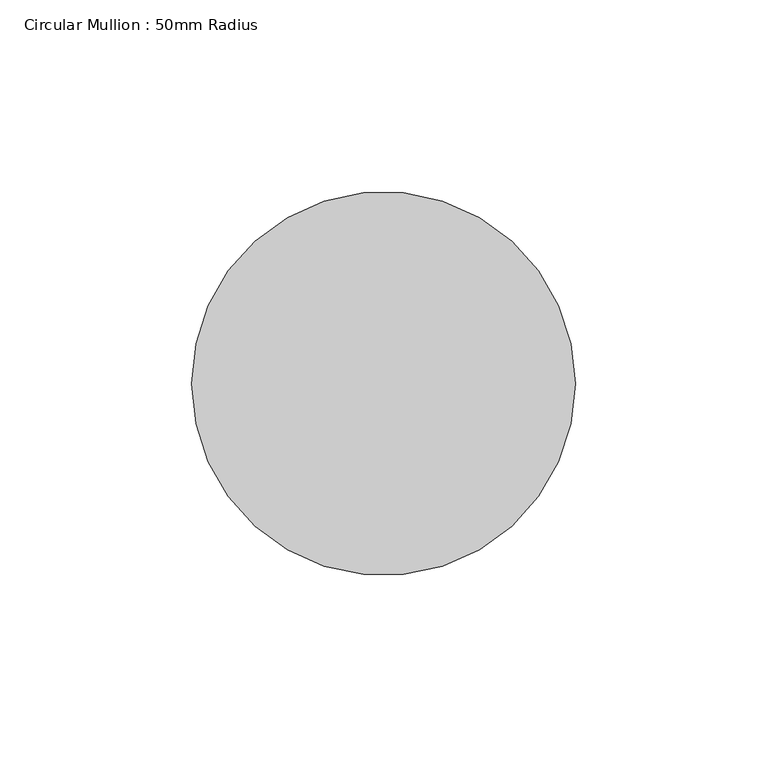
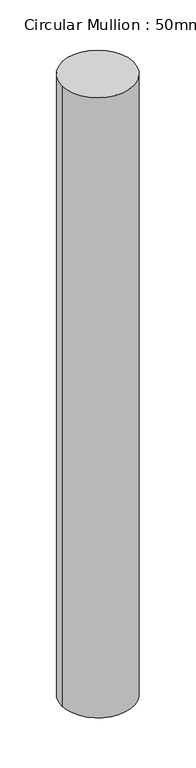
"""IFC4 building model written with IfcOpenShell, lengths in millimetres: member geometry, Circular Mullion : 50mm Radius."""

import ifcopenshell
import ifcopenshell.guid

model = None  # the IFC model being written
_history = None  # IfcOwnerHistory: only IFC2X3 demands one
_inside = {}  # id of a spatial element -> (the spatial element, [elements in it])
_under = {}  # id of a project, library or spatial element -> (it, [spatial elements below it])
_declared = {}  # id of a project -> (the project, [libraries it declares])
_typed = {}  # id of a type object -> (the type object, [elements of that type])
_made_of = {}  # id of a material, layer set ... -> (it, [elements and type objects made of it])


def new_model(schema):
    """Start an empty IFC model of exactly this schema.

    Asked for "IFC4X3", IfcOpenShell would pick the latest addendum, in which some entities
    have other attributes; the version numbers below select the first issue.
    IFC2X3 requires an IfcOwnerHistory on every rooted entity: one is made here for all.
    """
    global model, _history
    if schema == "IFC4X3":
        model = ifcopenshell.file(schema_version=(4, 3, 0, 0))
    else:
        model = ifcopenshell.file(schema=schema)
    _inside.clear()
    _under.clear()
    _declared.clear()
    _typed.clear()
    _made_of.clear()
    _history = None
    if model.schema == "IFC2X3":
        org = make("IfcOrganization", Name="unknown")
        user = make(
            "IfcPersonAndOrganization",
            ThePerson=make("IfcPerson", FamilyName="unknown"),
            TheOrganization=org,
        )
        app = make(
            "IfcApplication",
            ApplicationDeveloper=org,
            Version="unknown",
            ApplicationFullName="unknown",
            ApplicationIdentifier="unknown",
        )
        _history = make(
            "IfcOwnerHistory",
            OwningUser=user,
            OwningApplication=app,
            ChangeAction="ADDED",
            CreationDate=0,
        )
    return model


def make(cls, **values):
    """One entity of the class cls with the attributes given. An attribute that is None is left unset."""
    return model.create_entity(
        cls, **{name: value for name, value in values.items() if value is not None}
    )


def rooted(cls, **values):
    """An entity with a GlobalId (a new one), such as an element, a storey or a relation."""
    return make(cls, GlobalId=ifcopenshell.guid.new(), OwnerHistory=_history, **values)


def si_unit(unit_type, name, prefix=None):
    """IfcSIUnit, for example si_unit("LENGTHUNIT", "METRE", prefix="MILLI")."""
    return make("IfcSIUnit", UnitType=unit_type, Prefix=prefix, Name=name)


def assignment(units):
    """IfcUnitAssignment: the units of a project."""
    return None if units is None else make("IfcUnitAssignment", Units=units)


def point(xyz):
    """IfcCartesianPoint."""
    return None if xyz is None else make("IfcCartesianPoint", Coordinates=xyz)


def direction(xyz):
    """IfcDirection."""
    return None if xyz is None else make("IfcDirection", DirectionRatios=xyz)


def frame(location, z_axis=None, x_axis=None):
    """IfcAxis2Placement3D, a coordinate frame: its origin and axes. An axis left out is left unset."""
    return make(
        "IfcAxis2Placement3D",
        Location=point(location),
        Axis=direction(z_axis),
        RefDirection=direction(x_axis),
    )


def frame_2d(location, x_axis=None):
    """IfcAxis2Placement2D, a coordinate frame in the plane: its origin and x axis."""
    return make(
        "IfcAxis2Placement2D", Location=point(location), RefDirection=direction(x_axis)
    )


def origin():
    """The frame at (0, 0, 0) with its axes left unset."""
    return frame((0.0, 0.0, 0.0))


def origin_2d():
    """The frame at (0, 0) in the plane with its x axis left unset."""
    return frame_2d((0.0, 0.0))


def place(relative_to, where):
    """IfcLocalPlacement: puts the frame where relative to a parent placement (None: the world)."""
    return make(
        "IfcLocalPlacement", PlacementRelTo=relative_to, RelativePlacement=where
    )


def context(
    kind, dimensions, precision=None, world=None, true_north=None, identifier=None
):
    """IfcGeometricRepresentationContext, for example the 3D "Model" context."""
    return make(
        "IfcGeometricRepresentationContext",
        ContextIdentifier=identifier,
        ContextType=kind,
        CoordinateSpaceDimension=dimensions,
        Precision=precision,
        WorldCoordinateSystem=world,
        TrueNorth=true_north,
    )


def project(units=None, contexts=None):
    """IfcProject with its units and contexts."""
    return rooted(
        "IfcProject",
        Name="project",
        RepresentationContexts=contexts,
        UnitsInContext=assignment(units),
    )


def spatial(cls, under=None, at=None, **own):
    """A site, building, storey or space (cls), placed at a placement, below another one or the project."""
    s = rooted(cls, ObjectPlacement=at, **own)
    if under is not None:
        _under.setdefault(under.id(), (under, []))[1].append(s)
    return s


def circle_curve(where, radius):
    """IfcCircle in the frame where."""
    return make("IfcCircle", Position=where, Radius=radius)


def trimmed(basis, trim1, trim2, sense, master):
    """IfcTrimmedCurve: the piece of a basis curve between two trims."""
    return make(
        "IfcTrimmedCurve",
        BasisCurve=basis,
        Trim1=trim1,
        Trim2=trim2,
        SenseAgreement=sense,
        MasterRepresentation=master,
    )


def segment(curve, same_sense, transition):
    """IfcCompositeCurveSegment."""
    return make(
        "IfcCompositeCurveSegment",
        Transition=transition,
        SameSense=same_sense,
        ParentCurve=curve,
    )


def composite_curve(segments, self_intersect=None):
    """IfcCompositeCurve: segments joined end to end."""
    return make("IfcCompositeCurve", Segments=segments, SelfIntersect=self_intersect)


def outline(outer, holes=None, kind="AREA"):
    """IfcArbitraryClosedProfileDef: a profile drawn as a closed curve; with holes, ...WithVoids."""
    if holes is None:
        return make("IfcArbitraryClosedProfileDef", ProfileType=kind, OuterCurve=outer)
    return make(
        "IfcArbitraryProfileDefWithVoids",
        ProfileType=kind,
        OuterCurve=outer,
        InnerCurves=holes,
    )


def extrude(swept, where, along, depth):
    """IfcExtrudedAreaSolid: the profile swept, set in the frame where, extruded along a direction by depth."""
    return make(
        "IfcExtrudedAreaSolid",
        SweptArea=swept,
        Position=where,
        ExtrudedDirection=direction(along),
        Depth=depth,
    )


def shape(context_of_items, identifier, shape_type, items):
    """IfcShapeRepresentation: the items that make up one representation, for example the "Body"."""
    return make(
        "IfcShapeRepresentation",
        ContextOfItems=context_of_items,
        RepresentationIdentifier=identifier,
        RepresentationType=shape_type,
        Items=items,
    )


def source(mapping_origin, context_of_items, identifier, shape_type, items):
    """IfcRepresentationMap: a shape defined once, which mapped items show again and again."""
    return make(
        "IfcRepresentationMap",
        MappingOrigin=mapping_origin,
        MappedRepresentation=shape(context_of_items, identifier, shape_type, items),
    )


def transform(
    local_origin,
    x_axis=None,
    y_axis=None,
    z_axis=None,
    scale=None,
    scale2=None,
    scale3=None,
    uniform=True,
):
    """IfcCartesianTransformationOperator3D, or its non-uniform kind. x_axis, y_axis, z_axis: its Axis1, 2, 3."""
    if uniform:
        return make(
            "IfcCartesianTransformationOperator3D",
            Axis1=direction(x_axis),
            Axis2=direction(y_axis),
            LocalOrigin=point(local_origin),
            Scale=scale,
            Axis3=direction(z_axis),
        )
    return make(
        "IfcCartesianTransformationOperator3DnonUniform",
        Axis1=direction(x_axis),
        Axis2=direction(y_axis),
        LocalOrigin=point(local_origin),
        Scale=scale,
        Axis3=direction(z_axis),
        Scale2=scale2,
        Scale3=scale3,
    )


def mapped(mapping_source, mapping_target):
    """IfcMappedItem: shows the shape of a source again, moved by a transform."""
    return make(
        "IfcMappedItem", MappingSource=mapping_source, MappingTarget=mapping_target
    )


def made_of(thing, what):
    """Note that an element or type object is made of a material, layer set ...; save() writes the relation."""
    if what is not None:
        _made_of.setdefault(what.id(), (what, []))[1].append(thing)
    return thing


def element(
    cls,
    number,
    at=None,
    inside=None,
    cuts=None,
    type_object=None,
    material=None,
    context=None,
    identifier="Body",
    shape_type=None,
    held_by="IfcProductDefinitionShape",
    body=None,
    shapes=None,
    **own,
):
    """One element of the class cls, such as IfcWall. Its Tag is "e" and its number.

    at: its placement. inside: the storey or other place that contains it. cuts: it is an
    opening in that element (IfcRelVoidsElement). A single representation is given by context,
    identifier, shape_type and body (its items); several are given by shapes. held_by: the class
    of the entity that holds the representations. save() writes the other relations.
    """
    e = rooted(cls, Tag="e%d" % number, ObjectPlacement=at, **own)
    if body is not None:
        shapes = [shape(context, identifier, shape_type, body)]
    if shapes is not None:
        e.Representation = make(held_by, Representations=shapes)
    if inside is not None:
        _inside.setdefault(inside.id(), (inside, []))[1].append(e)
    if cuts is not None:
        rooted(
            "IfcRelVoidsElement", RelatingBuildingElement=cuts, RelatedOpeningElement=e
        )
    if type_object is not None:
        _typed.setdefault(type_object.id(), (type_object, []))[1].append(e)
    return made_of(e, material)


def aggregate(whole, parts):
    """IfcRelAggregates: a whole, such as a stair, and the parts it consists of."""
    return rooted("IfcRelAggregates", RelatingObject=whole, RelatedObjects=parts)


def save(model, path):
    """Write the relations noted so far, then the file.

    IfcRelAggregates (storeys below a building ...), IfcRelContainedInSpatialStructure (elements
    in a storey), IfcRelDefinesByType, IfcRelAssociatesMaterial and IfcRelDeclares: one each for
    every whole, place, type object, material and project.
    """
    for whole, parts in _under.values():
        aggregate(whole, parts)
    for where, things in _inside.values():
        rooted(
            "IfcRelContainedInSpatialStructure",
            RelatedElements=things,
            RelatingStructure=where,
        )
    for kind, things in _typed.values():
        rooted("IfcRelDefinesByType", RelatedObjects=things, RelatingType=kind)
    for what, things in _made_of.values():
        rooted("IfcRelAssociatesMaterial", RelatedObjects=things, RelatingMaterial=what)
    for by, libraries in _declared.values():
        rooted("IfcRelDeclares", RelatingContext=by, RelatedDefinitions=libraries)
    model.write(path)


def circular_mullion_50mm_radius_4a2e5ca3(model_context):
    return source(origin(), model_context, "Body", "SweptSolid", [
        extrude(outline(composite_curve([segment(trimmed(circle_curve(origin_2d(), 50.0), [point((50.0, 0.0))], [point((-50.0, 0.0))], False, "CARTESIAN"), True, "CONTINUOUS"), segment(trimmed(circle_curve(origin_2d(), 50.0), [point((-50.0, 0.0))], [point((50.0, 0.0))], False, "CARTESIAN"), True, "CONTINUOUS")], self_intersect=False)), frame((0.0, 0.0, -914.0074423), z_axis=(0.0, 0.0, 1.0), x_axis=(1.0, 0.0, 0.0)), (0.0, 0.0, 1.0), 914.0074423),
    ])


if __name__ == "__main__":
    model = new_model("IFC4")
    model_context = context("Model", 3, world=origin())
    ifc_project = project(units=[si_unit("LENGTHUNIT", "METRE", prefix="MILLI")], contexts=[model_context])
    site = spatial("IfcSite", under=ifc_project)
    building = spatial("IfcBuilding", under=site)
    placement = place(None, origin())
    circular_mullion_50mm_radius_shape = circular_mullion_50mm_radius_4a2e5ca3(model_context)
    element("IfcMember", 1, ObjectType="Circular Mullion : 50mm Radius", at=placement, inside=building, context=model_context, shape_type="MappedRepresentation", body=[
        mapped(circular_mullion_50mm_radius_shape, transform((0.0, 0.0, 0.0), x_axis=(1.0, 0.0, 0.0), y_axis=(0.0, 1.0, 0.0), z_axis=(0.0, 0.0, 1.0))),
    ])
    save(model, "model.ifc")

# Revit data of these elements
# Type "Circular Mullion : 50mm Radius"
#   built-in parameter 1007350 = 0.164042 (stored number, unit not read)
# Element 1 (IfcMember, "Circular Mullion : 50mm Radius")
#   Materials on its faces: "Aluminium"
# Materials
#   "Aluminium": class "Metal", colour RGB 247 247 247, transparency 0, Description = "Aluminium 6061", Cost = 0
